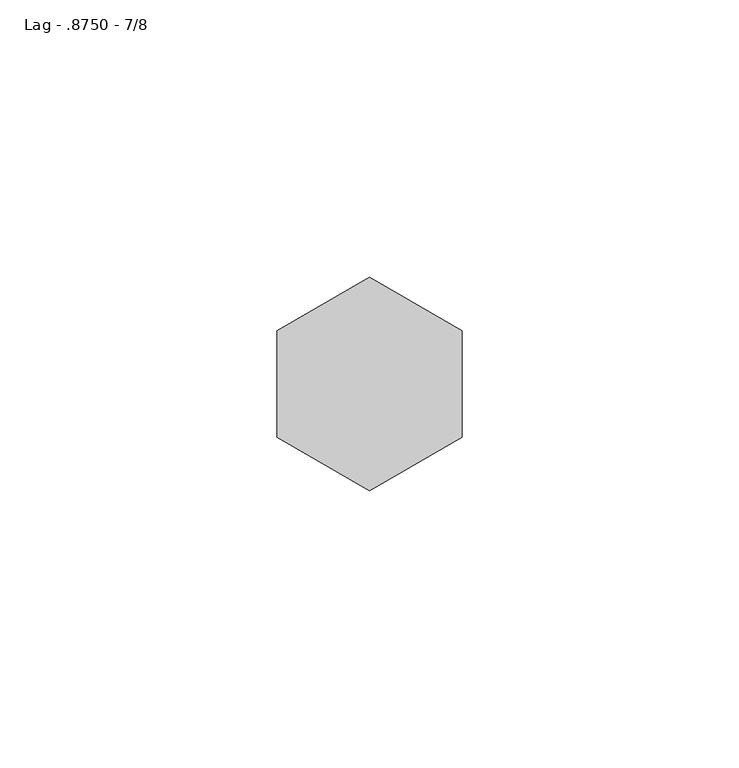
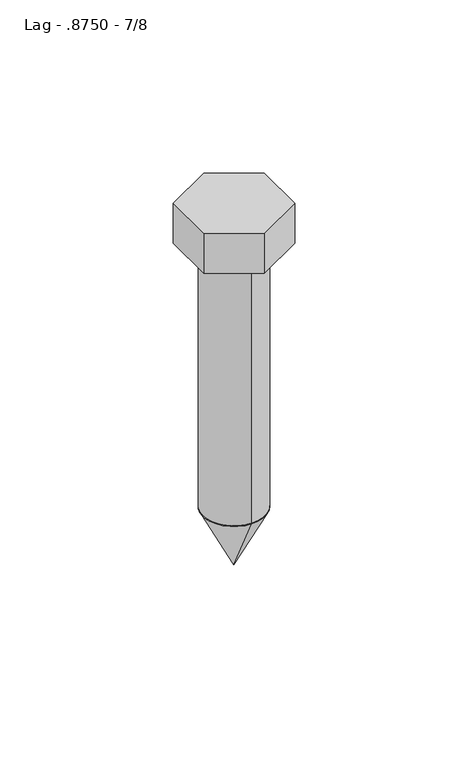
"""IFC4 building model written with IfcOpenShell, lengths in millimetres: fastener geometry, 060523 - W_P_C - Fastenings - Generic : Lag - .8750 - 7/8."""

from ifc_helpers import new_model, si_unit, point, frame, origin, origin_with_axes, origin_2d, place, context, project, spatial, polyline, circle_curve, trimmed, segment, composite_curve, outline, extrude, source, transform, mapped, element, save
from ifc_brep_helpers import plane_surface, revolved_surface, advanced_brep


def lag_8750_7_8_8902ef38(model_context):
    return source(origin(), model_context, "Body", "SolidModel", [
        advanced_brep(
        [(0.0, -11.3605469, -101.6), (0.0, 11.3605469, -101.6), (0.0, 0.0, -101.6), (0.0, 0.0, -124.3210937)],
        [
            (0, 1, circle_curve(frame((0.0, 0.0, -101.6), z_axis=(0.0, 0.0, 1.0), x_axis=(0.0, 1.0, 0.0)), 11.3605469)),
            (1, 2),
            (2, 0),
            (1, 0, circle_curve(frame((0.0, 0.0, -101.6), z_axis=(0.0, 0.0, 1.0), x_axis=(0.0, 1.0, 0.0)), 11.3605469)),
            (3, 1),
            (0, 3),
        ],
        [
            plane_surface(frame((0.0, 0.0, -101.6), z_axis=(0.0, 0.0, 1.0), x_axis=(0.0, 1.0, 0.0))),
            revolved_surface(polyline([(0.0, 11.3605469, -101.6), (0.0, 0.0, -124.3210937)]), (0.0, 0.0, -103.0840259), (0.0, 0.0, -1.0)),
        ],
        [
            (0, [[1, 2, 3]]),
            (0, [[4, -3, -2]]),
            (1, [[5, -1, 6]]),
            (1, [[-6, -4, -5]]),
        ],
    ),
        extrude(outline(polyline([(-16.66875, 9.6237073), (0.0, 19.2474146), (16.66875, 9.6237073), (16.66875, -9.6237073), (0.0, -19.2474146), (-16.66875, -9.6237073), (-16.66875, 9.6237073)])), origin_with_axes(), (0.0, 0.0, 1.0), 15.3789062),
        extrude(outline(composite_curve([segment(trimmed(circle_curve(origin_2d(), 11.3605469), [point((0.0, -11.3605469))], [point((0.0, 11.3605469))], False, "CARTESIAN"), True, "CONTINUOUS"), segment(trimmed(circle_curve(origin_2d(), 11.3605469), [point((0.0, 11.3605469))], [point((0.0, -11.3605469))], False, "CARTESIAN"), True, "CONTINUOUS")], self_intersect=False)), frame((0.0, 0.0, -101.6), z_axis=(0.0, 0.0, 1.0), x_axis=(1.0, 0.0, 0.0)), (0.0, 0.0, 1.0), 101.6),
    ])


if __name__ == "__main__":
    model = new_model("IFC4")
    model_context = context("Model", 3, world=origin())
    ifc_project = project(units=[si_unit("LENGTHUNIT", "METRE", prefix="MILLI")], contexts=[model_context])
    site = spatial("IfcSite", under=ifc_project)
    building = spatial("IfcBuilding", under=site)
    placement = place(None, origin())
    lag_8750_7_8_shape = lag_8750_7_8_8902ef38(model_context)
    element("IfcFastener", 1, ObjectType="060523 - W_P_C - Fastenings - Generic : Lag - .8750 - 7/8", at=placement, inside=building, context=model_context, shape_type="MappedRepresentation", body=[
        mapped(lag_8750_7_8_shape, transform((0.0, 0.0, 0.0), x_axis=(1.0, 0.0, 0.0), y_axis=(0.0, 1.0, 0.0), z_axis=(0.0, 0.0, 1.0))),
    ])
    save(model, "model.ifc")

# Revit data of these elements
# Type "060523 - W_P_C - Fastenings - Generic : Lag - .8750 - 7/8"
#   Washer_Thickness = 0' - 0.20182"
#   Washer Radius = 0' - 1.05273"
#   Washer Offset - Head = 0' - 0"
#   Washer Offset = 0' - 0"
#   Thickness_of_Substrate [instance default] = 0' - 1"
#   Side = 0' - 0.75879"
#   Radius = 0' - 0.44727"
#   Length [instance default] = 0' - 4"
#   Head Size = 0' - 1 5/16"
#   Head Radius = 0' - 0 21/32"
#   Head Height = 0' - 0 155/256"
#   Double Diameter = 0' - 1 101/128"
#   Diameter = 0' - 0 229/256"
#   Default Elevation = 4' - 0"
#   Washer_Nut_Visibility = no
#   Washer_Head_Visibility = no
#   Round_Head_Visibility = no
#   Point Visibility = yes
#   Nut_Visibility = no
#   Hex_Head_Visiblilty = yes
#   Washer Material = none
#   Bolt Material (Size) = AT SILL - FASTENER AT 24" O.C.
# Element 1 (IfcFastener, "060523 - W_P_C - Fastenings - Generic : Lag - .8750 - 7/8")
#   Materials on its faces: "AT SILL - FASTENER AT 24\" O.C."
# Materials
#   "AT SILL - FASTENER AT 24\" O.C.": class "Generic", colour RGB 120 120 120, transparency 0, Cost = 0
